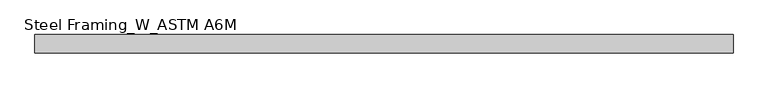
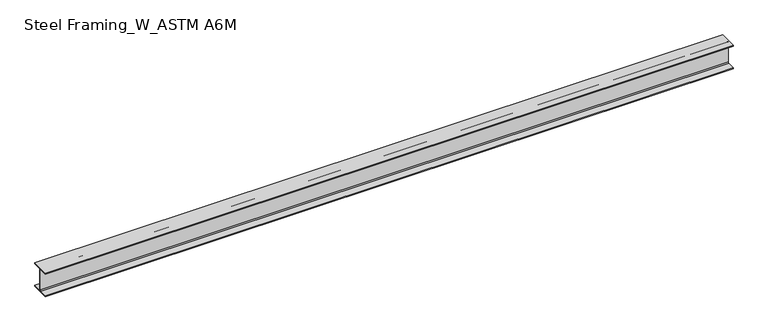
"""IFC4 building model written with IfcOpenShell, lengths in millimetres: beam geometry, Steel Framing_W_ASTM A6M : H_SB_AR_S02_W360x91_B3."""

import ifcopenshell
import ifcopenshell.guid

model = None  # the IFC model being written
_history = None  # IfcOwnerHistory: only IFC2X3 demands one
_inside = {}  # id of a spatial element -> (the spatial element, [elements in it])
_under = {}  # id of a project, library or spatial element -> (it, [spatial elements below it])
_declared = {}  # id of a project -> (the project, [libraries it declares])
_typed = {}  # id of a type object -> (the type object, [elements of that type])
_made_of = {}  # id of a material, layer set ... -> (it, [elements and type objects made of it])


def new_model(schema):
    """Start an empty IFC model of exactly this schema.

    Asked for "IFC4X3", IfcOpenShell would pick the latest addendum, in which some entities
    have other attributes; the version numbers below select the first issue.
    IFC2X3 requires an IfcOwnerHistory on every rooted entity: one is made here for all.
    """
    global model, _history
    if schema == "IFC4X3":
        model = ifcopenshell.file(schema_version=(4, 3, 0, 0))
    else:
        model = ifcopenshell.file(schema=schema)
    _inside.clear()
    _under.clear()
    _declared.clear()
    _typed.clear()
    _made_of.clear()
    _history = None
    if model.schema == "IFC2X3":
        org = make("IfcOrganization", Name="unknown")
        user = make(
            "IfcPersonAndOrganization",
            ThePerson=make("IfcPerson", FamilyName="unknown"),
            TheOrganization=org,
        )
        app = make(
            "IfcApplication",
            ApplicationDeveloper=org,
            Version="unknown",
            ApplicationFullName="unknown",
            ApplicationIdentifier="unknown",
        )
        _history = make(
            "IfcOwnerHistory",
            OwningUser=user,
            OwningApplication=app,
            ChangeAction="ADDED",
            CreationDate=0,
        )
    return model


def make(cls, **values):
    """One entity of the class cls with the attributes given. An attribute that is None is left unset."""
    return model.create_entity(
        cls, **{name: value for name, value in values.items() if value is not None}
    )


def rooted(cls, **values):
    """An entity with a GlobalId (a new one), such as an element, a storey or a relation."""
    return make(cls, GlobalId=ifcopenshell.guid.new(), OwnerHistory=_history, **values)


def si_unit(unit_type, name, prefix=None):
    """IfcSIUnit, for example si_unit("LENGTHUNIT", "METRE", prefix="MILLI")."""
    return make("IfcSIUnit", UnitType=unit_type, Prefix=prefix, Name=name)


def assignment(units):
    """IfcUnitAssignment: the units of a project."""
    return None if units is None else make("IfcUnitAssignment", Units=units)


def point(xyz):
    """IfcCartesianPoint."""
    return None if xyz is None else make("IfcCartesianPoint", Coordinates=xyz)


def direction(xyz):
    """IfcDirection."""
    return None if xyz is None else make("IfcDirection", DirectionRatios=xyz)


def frame(location, z_axis=None, x_axis=None):
    """IfcAxis2Placement3D, a coordinate frame: its origin and axes. An axis left out is left unset."""
    return make(
        "IfcAxis2Placement3D",
        Location=point(location),
        Axis=direction(z_axis),
        RefDirection=direction(x_axis),
    )


def frame_2d(location, x_axis=None):
    """IfcAxis2Placement2D, a coordinate frame in the plane: its origin and x axis."""
    return make(
        "IfcAxis2Placement2D", Location=point(location), RefDirection=direction(x_axis)
    )


def origin():
    """The frame at (0, 0, 0) with its axes left unset."""
    return frame((0.0, 0.0, 0.0))


def place(relative_to, where):
    """IfcLocalPlacement: puts the frame where relative to a parent placement (None: the world)."""
    return make(
        "IfcLocalPlacement", PlacementRelTo=relative_to, RelativePlacement=where
    )


def context(
    kind, dimensions, precision=None, world=None, true_north=None, identifier=None
):
    """IfcGeometricRepresentationContext, for example the 3D "Model" context."""
    return make(
        "IfcGeometricRepresentationContext",
        ContextIdentifier=identifier,
        ContextType=kind,
        CoordinateSpaceDimension=dimensions,
        Precision=precision,
        WorldCoordinateSystem=world,
        TrueNorth=true_north,
    )


def project(units=None, contexts=None):
    """IfcProject with its units and contexts."""
    return rooted(
        "IfcProject",
        Name="project",
        RepresentationContexts=contexts,
        UnitsInContext=assignment(units),
    )


def spatial(cls, under=None, at=None, **own):
    """A site, building, storey or space (cls), placed at a placement, below another one or the project."""
    s = rooted(cls, ObjectPlacement=at, **own)
    if under is not None:
        _under.setdefault(under.id(), (under, []))[1].append(s)
    return s


def polyline(points):
    """IfcPolyline through the points."""
    return make("IfcPolyline", Points=[point(p) for p in points])


def circle_curve(where, radius):
    """IfcCircle in the frame where."""
    return make("IfcCircle", Position=where, Radius=radius)


def trimmed(basis, trim1, trim2, sense, master):
    """IfcTrimmedCurve: the piece of a basis curve between two trims."""
    return make(
        "IfcTrimmedCurve",
        BasisCurve=basis,
        Trim1=trim1,
        Trim2=trim2,
        SenseAgreement=sense,
        MasterRepresentation=master,
    )


def segment(curve, same_sense, transition):
    """IfcCompositeCurveSegment."""
    return make(
        "IfcCompositeCurveSegment",
        Transition=transition,
        SameSense=same_sense,
        ParentCurve=curve,
    )


def composite_curve(segments, self_intersect=None):
    """IfcCompositeCurve: segments joined end to end."""
    return make("IfcCompositeCurve", Segments=segments, SelfIntersect=self_intersect)


def outline(outer, holes=None, kind="AREA"):
    """IfcArbitraryClosedProfileDef: a profile drawn as a closed curve; with holes, ...WithVoids."""
    if holes is None:
        return make("IfcArbitraryClosedProfileDef", ProfileType=kind, OuterCurve=outer)
    return make(
        "IfcArbitraryProfileDefWithVoids",
        ProfileType=kind,
        OuterCurve=outer,
        InnerCurves=holes,
    )


def extrude(swept, where, along, depth):
    """IfcExtrudedAreaSolid: the profile swept, set in the frame where, extruded along a direction by depth."""
    return make(
        "IfcExtrudedAreaSolid",
        SweptArea=swept,
        Position=where,
        ExtrudedDirection=direction(along),
        Depth=depth,
    )


def shape(context_of_items, identifier, shape_type, items):
    """IfcShapeRepresentation: the items that make up one representation, for example the "Body"."""
    return make(
        "IfcShapeRepresentation",
        ContextOfItems=context_of_items,
        RepresentationIdentifier=identifier,
        RepresentationType=shape_type,
        Items=items,
    )


def source(mapping_origin, context_of_items, identifier, shape_type, items):
    """IfcRepresentationMap: a shape defined once, which mapped items show again and again."""
    return make(
        "IfcRepresentationMap",
        MappingOrigin=mapping_origin,
        MappedRepresentation=shape(context_of_items, identifier, shape_type, items),
    )


def transform(
    local_origin,
    x_axis=None,
    y_axis=None,
    z_axis=None,
    scale=None,
    scale2=None,
    scale3=None,
    uniform=True,
):
    """IfcCartesianTransformationOperator3D, or its non-uniform kind. x_axis, y_axis, z_axis: its Axis1, 2, 3."""
    if uniform:
        return make(
            "IfcCartesianTransformationOperator3D",
            Axis1=direction(x_axis),
            Axis2=direction(y_axis),
            LocalOrigin=point(local_origin),
            Scale=scale,
            Axis3=direction(z_axis),
        )
    return make(
        "IfcCartesianTransformationOperator3DnonUniform",
        Axis1=direction(x_axis),
        Axis2=direction(y_axis),
        LocalOrigin=point(local_origin),
        Scale=scale,
        Axis3=direction(z_axis),
        Scale2=scale2,
        Scale3=scale3,
    )


def mapped(mapping_source, mapping_target):
    """IfcMappedItem: shows the shape of a source again, moved by a transform."""
    return make(
        "IfcMappedItem", MappingSource=mapping_source, MappingTarget=mapping_target
    )


def made_of(thing, what):
    """Note that an element or type object is made of a material, layer set ...; save() writes the relation."""
    if what is not None:
        _made_of.setdefault(what.id(), (what, []))[1].append(thing)
    return thing


def element(
    cls,
    number,
    at=None,
    inside=None,
    cuts=None,
    type_object=None,
    material=None,
    context=None,
    identifier="Body",
    shape_type=None,
    held_by="IfcProductDefinitionShape",
    body=None,
    shapes=None,
    **own,
):
    """One element of the class cls, such as IfcWall. Its Tag is "e" and its number.

    at: its placement. inside: the storey or other place that contains it. cuts: it is an
    opening in that element (IfcRelVoidsElement). A single representation is given by context,
    identifier, shape_type and body (its items); several are given by shapes. held_by: the class
    of the entity that holds the representations. save() writes the other relations.
    """
    e = rooted(cls, Tag="e%d" % number, ObjectPlacement=at, **own)
    if body is not None:
        shapes = [shape(context, identifier, shape_type, body)]
    if shapes is not None:
        e.Representation = make(held_by, Representations=shapes)
    if inside is not None:
        _inside.setdefault(inside.id(), (inside, []))[1].append(e)
    if cuts is not None:
        rooted(
            "IfcRelVoidsElement", RelatingBuildingElement=cuts, RelatedOpeningElement=e
        )
    if type_object is not None:
        _typed.setdefault(type_object.id(), (type_object, []))[1].append(e)
    return made_of(e, material)


def aggregate(whole, parts):
    """IfcRelAggregates: a whole, such as a stair, and the parts it consists of."""
    return rooted("IfcRelAggregates", RelatingObject=whole, RelatedObjects=parts)


def save(model, path):
    """Write the relations noted so far, then the file.

    IfcRelAggregates (storeys below a building ...), IfcRelContainedInSpatialStructure (elements
    in a storey), IfcRelDefinesByType, IfcRelAssociatesMaterial and IfcRelDeclares: one each for
    every whole, place, type object, material and project.
    """
    for whole, parts in _under.values():
        aggregate(whole, parts)
    for where, things in _inside.values():
        rooted(
            "IfcRelContainedInSpatialStructure",
            RelatedElements=things,
            RelatingStructure=where,
        )
    for kind, things in _typed.values():
        rooted("IfcRelDefinesByType", RelatedObjects=things, RelatingType=kind)
    for what, things in _made_of.values():
        rooted("IfcRelAssociatesMaterial", RelatedObjects=things, RelatingMaterial=what)
    for by, libraries in _declared.values():
        rooted("IfcRelDeclares", RelatingContext=by, RelatedDefinitions=libraries)
    model.write(path)


def steel_framing_w_astm_a6m_17837fc5(model_context):
    return source(origin(), model_context, "Body", "SweptSolid", [
        extrude(outline(composite_curve([segment(polyline([(127.0, -160.1), (127.0, -176.5), (-127.0, -176.5), (-127.0, -160.1), (-19.865, -160.1)]), True, "CONTINUOUS"), segment(trimmed(circle_curve(frame_2d((-19.865, -145.0)), 15.1), [point((-19.865, -160.1))], [point((-4.765, -145.0))], True, "CARTESIAN"), True, "CONTINUOUS"), segment(polyline([(-4.765, -145.0), (-4.765, 145.0)]), True, "CONTINUOUS"), segment(trimmed(circle_curve(frame_2d((-19.865, 145.0)), 15.1), [point((-4.765, 145.0))], [point((-19.865, 160.1))], True, "CARTESIAN"), True, "CONTINUOUS"), segment(polyline([(-19.865, 160.1), (-127.0, 160.1), (-127.0, 176.5), (127.0, 176.5), (127.0, 160.1), (19.865, 160.1)]), True, "CONTINUOUS"), segment(trimmed(circle_curve(frame_2d((19.865, 145.0)), 15.1), [point((19.865, 160.1))], [point((4.765, 145.0))], True, "CARTESIAN"), True, "CONTINUOUS"), segment(polyline([(4.765, 145.0), (4.765, -145.0)]), True, "CONTINUOUS"), segment(trimmed(circle_curve(frame_2d((19.865, -145.0)), 15.1), [point((4.765, -145.0))], [point((19.865, -160.1))], True, "CARTESIAN"), True, "CONTINUOUS"), segment(polyline([(19.865, -160.1), (127.0, -160.1)]), True, "CONTINUOUS")], self_intersect=False)), frame((-4846.3, 0.0, 0.0), z_axis=(1.0, 0.0, 0.0), x_axis=(0.0, 1.0, 0.0)), (0.0, 0.0, 1.0), 9692.6),
    ])


if __name__ == "__main__":
    model = new_model("IFC4")
    model_context = context("Model", 3, world=origin())
    ifc_project = project(units=[si_unit("LENGTHUNIT", "METRE", prefix="MILLI")], contexts=[model_context])
    site = spatial("IfcSite", under=ifc_project)
    building = spatial("IfcBuilding", under=site)
    placement = place(None, origin())
    steel_framing_w_astm_a6m_shape = steel_framing_w_astm_a6m_17837fc5(model_context)
    element("IfcBeam", 1, ObjectType="Steel Framing_W_ASTM A6M : H_SB_AR_S02_W360x91_B3", at=placement, inside=building, context=model_context, shape_type="MappedRepresentation", body=[
        mapped(steel_framing_w_astm_a6m_shape, transform((0.0, 0.0, 0.0), x_axis=(1.0, 0.0, 0.0), y_axis=(0.0, 1.0, 0.0), z_axis=(0.0, 0.0, 1.0))),
    ])
    save(model, "model.ifc")

# Revit data of these elements
# Type "Steel Framing_W_ASTM A6M : H_SB_AR_S02_W360x91_B3"
#   Type Mark = "B3"
#   Section Name Key = "W14x61"
#   Width = 25.4 cm
#   Web Thickness = 0.953 cm
#   Web Fillet = 1.51 cm
#   Warping Constant = 1260000.0 cm⁶
#   Torsional Moment of Inertia = 91.20 cm⁴
#   Section Area = 115.0 cm²
#   Plastic Modulus weak axis = 537.0 cm³
#   Plastic Modulus strong axis = 1670.0 cm³
#   Perimeter = 1.68 m²/m
#   Nominal Weight = 91.00 kgf/m
#   Moment of Inertia weak axis = 4450.00 cm⁴
#   Moment of Inertia strong axis = 26600.00 cm⁴
#   Height = 35.3 cm
#   Flange Thickness = 1.64 cm
#   Elastic Modulus weak axis = 352.0 cm³
#   Elastic Modulus strong axis = 1510.0 cm³
#   Centroid Vertical = 17.65 cm
#   Centroid Horizontal = 12.7 cm
#   Length [instance default] = 1500 mm
#   Structural Material [instance default] = Steel, 45-345
#   Bolt Spacing = 0
#   Assembly Code = ""
# Element 1 (IfcBeam, "Steel Framing_W_ASTM A6M : H_SB_AR_S02_W360x91_B3")
#   Materials on its faces: "Steel, 45-345"
# Materials
#   "Steel, 45-345": class "Metal", colour RGB 189 187 185, transparency 0, Description = "Steel 345 MPa", Cost = 0
